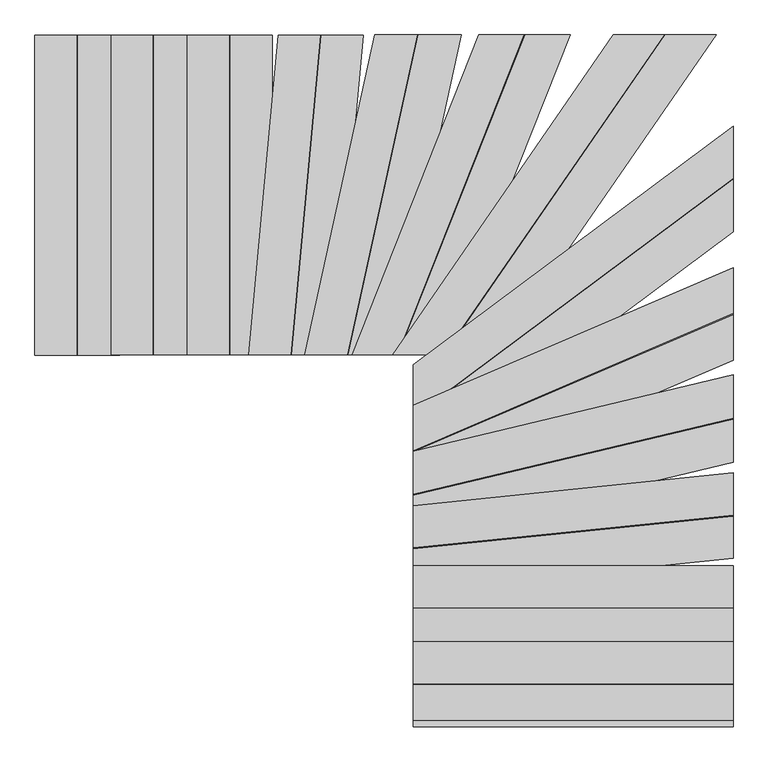
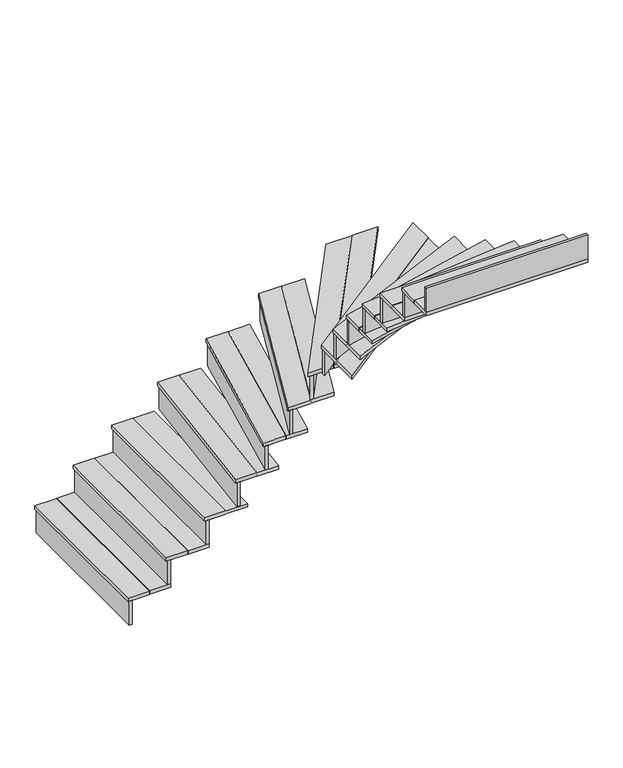
"""IFC4 building model written with IfcOpenShell, lengths in millimetres: stair flight geometry."""

from ifc_helpers import new_model, si_unit, origin, place, context, project, spatial, faceted_brep, source, transform, mapped, element, save


def stair_flight_5e1e636e(model_context):
    return source(origin(), model_context, "Body", "Brep", [
        faceted_brep([(-23979.400458, -9511.5570712, 168.402567), (-23979.400458, -9511.5570712, 0.0), (-23960.350458, -9511.5570712, 0.0), (-23960.350458, -9511.5570712, 168.402567), (-23979.400458, -8444.7570712, 168.402567), (-23960.350458, -8444.7570712, 168.402567), (-23960.350458, -8444.7570712, 0.0), (-23979.400458, -8444.7570712, 0.0)], [[[0, 1, 2, 3]], [[4, 5, 6, 7]], [[1, 0, 4, 7]], [[2, 1, 7, 6]], [[3, 2, 6, 5]], [[0, 3, 5, 4]]]),
        faceted_brep([(-23849.225458, -9511.5570712, 168.402567), (-23849.225458, -9511.5570712, 180.156839), (-23846.050458, -9511.5570712, 180.156839), (-23846.050458, -9511.5570712, 168.402567), (-23706.350458, -9511.5570712, 168.402567), (-23706.350458, -9511.5570712, 192.3142857), (-23846.050458, -9511.5570712, 192.3142857), (-23846.050458, -9511.5570712, 180.5600136), (-23849.225458, -9511.5570712, 180.5600136), (-23849.225458, -9511.5570712, 192.3142857), (-23988.925458, -9511.5570712, 192.3142857), (-23988.925458, -9511.5570712, 168.402567), (-23849.225458, -8444.7570712, 168.402567), (-23988.925458, -8444.7570712, 168.402567), (-23988.925458, -8444.7570712, 192.3142857), (-23849.225458, -8444.7570712, 192.3142857), (-23849.225458, -8444.7570712, 180.5600136), (-23846.050458, -8444.7570712, 180.5600136), (-23846.050458, -8444.7570712, 192.3142857), (-23706.350458, -8444.7570712, 192.3142857), (-23706.350458, -8444.7570712, 168.402567), (-23846.050458, -8444.7570712, 168.402567), (-23846.050458, -8444.7570712, 180.156839), (-23849.225458, -8444.7570712, 180.156839)], [[[0, 1, 2, 3, 4, 5, 6, 7, 8, 9, 10, 11]], [[12, 13, 14, 15, 16, 17, 18, 19, 20, 21, 22, 23]], [[1, 0, 12, 23]], [[2, 1, 23, 22]], [[3, 2, 22, 21]], [[4, 3, 21, 20]], [[5, 4, 20, 19]], [[6, 5, 19, 18]], [[7, 6, 18, 17]], [[8, 7, 17, 16]], [[9, 8, 16, 15]], [[10, 9, 15, 14]], [[11, 10, 14, 13]], [[0, 11, 13, 12]]]),
        faceted_brep([(-23725.400458, -9511.5570712, 360.7168527), (-23725.400458, -9511.5570712, 192.3142857), (-23706.350458, -9511.5570712, 192.3142857), (-23706.350458, -9511.5570712, 360.7168527), (-23725.400458, -8444.7570712, 360.7168527), (-23706.350458, -8444.7570712, 360.7168527), (-23706.350458, -8444.7570712, 192.3142857), (-23725.400458, -8444.7570712, 192.3142857)], [[[0, 1, 2, 3]], [[4, 5, 6, 7]], [[1, 0, 4, 7]], [[2, 1, 7, 6]], [[3, 2, 6, 5]], [[0, 3, 5, 4]]]),
        faceted_brep([(-23595.225458, -9511.5570712, 360.7168527), (-23595.225458, -9511.5570712, 372.4711248), (-23592.050458, -9511.5570712, 372.4711248), (-23592.050458, -9511.5570712, 360.7168527), (-23452.350458, -9511.5570712, 360.7168527), (-23452.350458, -9511.5570712, 384.6285714), (-23592.050458, -9511.5570712, 384.6285714), (-23592.050458, -9511.5570712, 372.8742994), (-23595.225458, -9511.5570712, 372.8742994), (-23595.225458, -9511.5570712, 384.6285714), (-23734.925458, -9511.5570712, 384.6285714), (-23734.925458, -9511.5570712, 360.7168527), (-23595.225458, -8444.7570712, 360.7168527), (-23734.925458, -8444.7570712, 360.7168527), (-23734.925458, -8444.7570712, 384.6285714), (-23595.225458, -8444.7570712, 384.6285714), (-23595.225458, -8444.7570712, 372.8742994), (-23592.050458, -8444.7570712, 372.8742994), (-23592.050458, -8444.7570712, 384.6285714), (-23452.350458, -8444.7570712, 384.6285714), (-23452.350458, -8444.7570712, 360.7168527), (-23592.050458, -8444.7570712, 360.7168527), (-23592.050458, -8444.7570712, 372.4711248), (-23595.225458, -8444.7570712, 372.4711248)], [[[0, 1, 2, 3, 4, 5, 6, 7, 8, 9, 10, 11]], [[12, 13, 14, 15, 16, 17, 18, 19, 20, 21, 22, 23]], [[1, 0, 12, 23]], [[2, 1, 23, 22]], [[3, 2, 22, 21]], [[4, 3, 21, 20]], [[5, 4, 20, 19]], [[6, 5, 19, 18]], [[7, 6, 18, 17]], [[8, 7, 17, 16]], [[9, 8, 16, 15]], [[10, 9, 15, 14]], [[11, 10, 14, 13]], [[0, 11, 13, 12]]]),
        faceted_brep([(-23471.400458, -9511.5570712, 553.0311384), (-23471.400458, -9511.5570712, 384.6285714), (-23452.350458, -9511.5570712, 384.6285714), (-23452.350458, -9511.5570712, 553.0311384), (-23471.400458, -8444.7570712, 553.0311384), (-23452.350458, -8444.7570712, 553.0311384), (-23452.350458, -8444.7570712, 384.6285714), (-23471.400458, -8444.7570712, 384.6285714)], [[[0, 1, 2, 3]], [[4, 5, 6, 7]], [[1, 0, 4, 7]], [[2, 1, 7, 6]], [[3, 2, 6, 5]], [[0, 3, 5, 4]]]),
        faceted_brep([(-23341.225458, -9511.5570712, 553.0311384), (-23341.225458, -9511.5570712, 564.7854105), (-23338.050458, -9511.5570712, 564.7854105), (-23338.050458, -9511.5570712, 553.0311384), (-23198.350458, -9511.5570712, 553.0311384), (-23198.350458, -9511.5570712, 576.9428571), (-23338.050458, -9511.5570712, 576.9428571), (-23338.050458, -9511.5570712, 565.1885851), (-23341.225458, -9511.5570712, 565.1885851), (-23341.225458, -9511.5570712, 576.9428571), (-23480.925458, -9511.5570712, 576.9428571), (-23480.925458, -9511.5570712, 553.0311384), (-23341.225458, -8444.7570712, 553.0311384), (-23480.925458, -8444.7570712, 553.0311384), (-23480.925458, -8444.7570712, 576.9428571), (-23341.225458, -8444.7570712, 576.9428571), (-23341.225458, -8444.7570712, 565.1885851), (-23338.050458, -8444.7570712, 565.1885851), (-23338.050458, -8444.7570712, 576.9428571), (-23198.350458, -8444.7570712, 576.9428571), (-23198.350458, -8444.7570712, 553.0311384), (-23338.050458, -8444.7570712, 553.0311384), (-23338.050458, -8444.7570712, 564.7854105), (-23341.225458, -8444.7570712, 564.7854105)], [[[0, 1, 2, 3, 4, 5, 6, 7, 8, 9, 10, 11]], [[12, 13, 14, 15, 16, 17, 18, 19, 20, 21, 22, 23]], [[1, 0, 12, 23]], [[2, 1, 23, 22]], [[3, 2, 22, 21]], [[4, 3, 21, 20]], [[5, 4, 20, 19]], [[6, 5, 19, 18]], [[7, 6, 18, 17]], [[8, 7, 17, 16]], [[9, 8, 16, 15]], [[10, 9, 15, 14]], [[11, 10, 14, 13]], [[0, 11, 13, 12]]]),
        faceted_brep([(-23267.1871269, -9511.5570712, 745.3454241), (-23267.1871269, -9511.5570712, 576.9428571), (-23248.0543246, -9511.5570712, 576.9428571), (-23248.0543246, -9511.5570712, 745.3454241), (-23167.6137891, -8444.7570712, 745.3454241), (-23148.4809868, -8444.7570712, 745.3454241), (-23148.4809868, -8444.7570712, 576.9428571), (-23167.6137891, -8444.7570712, 576.9428571)], [[[0, 1, 2, 3]], [[4, 5, 6, 7]], [[1, 0, 4, 7]], [[2, 1, 7, 6]], [[3, 2, 6, 5]], [[0, 3, 5, 4]]]),
        faceted_brep([(-23136.4463113, -9511.5570712, 745.3454241), (-23136.4463113, -9511.5570712, 757.0996962), (-23133.2575109, -9511.5570712, 757.0996962), (-23133.2575109, -9511.5570712, 745.3454241), (-22992.9502942, -9511.5570712, 745.3454241), (-22992.9502942, -9511.5570712, 769.2571429), (-23133.2575109, -9511.5570712, 769.2571429), (-23133.2575109, -9511.5570712, 757.5028708), (-23136.4463113, -9511.5570712, 757.5028708), (-23136.4463113, -9511.5570712, 769.2571429), (-23276.753528, -9511.5570712, 769.2571429), (-23276.753528, -9511.5570712, 745.3454241), (-23036.8729735, -8444.7570712, 745.3454241), (-23177.1801902, -8444.7570712, 745.3454241), (-23177.1801902, -8444.7570712, 769.2571429), (-23036.8729735, -8444.7570712, 769.2571429), (-23036.8729735, -8444.7570712, 757.5028708), (-23033.6841732, -8444.7570712, 757.5028708), (-23033.6841732, -8444.7570712, 769.2571429), (-22893.3769565, -8444.7570712, 769.2571429), (-22893.3769565, -8444.7570712, 745.3454241), (-23033.6841732, -8444.7570712, 745.3454241), (-23033.6841732, -8444.7570712, 757.0996962), (-23036.8729735, -8444.7570712, 757.0996962)], [[[0, 1, 2, 3, 4, 5, 6, 7, 8, 9, 10, 11]], [[12, 13, 14, 15, 16, 17, 18, 19, 20, 21, 22, 23]], [[1, 0, 12, 23]], [[2, 1, 23, 22]], [[3, 2, 22, 21]], [[4, 3, 21, 20]], [[5, 4, 20, 19]], [[6, 5, 19, 18]], [[7, 6, 18, 17]], [[8, 7, 17, 16]], [[9, 8, 16, 15]], [[10, 9, 15, 14]], [[11, 10, 14, 13]], [[0, 11, 13, 12]]]),
        faceted_brep([(-23080.0026813, -9511.5570712, 937.6597098), (-23080.0026813, -9511.5570712, 769.2571429), (-23060.502824, -9511.5570712, 769.2571429), (-23060.502824, -9511.5570712, 937.6597098), (-22846.7982346, -8444.7570712, 937.6597098), (-22827.2983773, -8444.7570712, 937.6597098), (-22827.2983773, -8444.7570712, 769.2571429), (-22846.7982346, -8444.7570712, 769.2571429)], [[[0, 1, 2, 3]], [[4, 5, 6, 7]], [[1, 0, 4, 7]], [[2, 1, 7, 6]], [[3, 2, 6, 5]], [[0, 3, 5, 4]]]),
        faceted_brep([(-22946.7536561, -9511.5570712, 937.6597098), (-22946.7536561, -9511.5570712, 949.4139819), (-22943.5036799, -9511.5570712, 949.4139819), (-22943.5036799, -9511.5570712, 937.6597098), (-22800.5047259, -9511.5570712, 937.6597098), (-22800.5047259, -9511.5570712, 961.5714286), (-22943.5036799, -9511.5570712, 961.5714286), (-22943.5036799, -9511.5570712, 949.8171565), (-22946.7536561, -9511.5570712, 949.8171565), (-22946.7536561, -9511.5570712, 961.5714286), (-23089.75261, -9511.5570712, 961.5714286), (-23089.75261, -9511.5570712, 937.6597098), (-22713.5492094, -8444.7570712, 937.6597098), (-22856.5481633, -8444.7570712, 937.6597098), (-22856.5481633, -8444.7570712, 961.5714286), (-22713.5492094, -8444.7570712, 961.5714286), (-22713.5492094, -8444.7570712, 949.8171565), (-22710.2992331, -8444.7570712, 949.8171565), (-22710.2992331, -8444.7570712, 961.5714286), (-22567.3002792, -8444.7570712, 961.5714286), (-22567.3002792, -8444.7570712, 937.6597098), (-22710.2992331, -8444.7570712, 937.6597098), (-22710.2992331, -8444.7570712, 949.4139819), (-22713.5492094, -8444.7570712, 949.4139819)], [[[0, 1, 2, 3, 4, 5, 6, 7, 8, 9, 10, 11]], [[12, 13, 14, 15, 16, 17, 18, 19, 20, 21, 22, 23]], [[1, 0, 12, 23]], [[2, 1, 23, 22]], [[3, 2, 22, 21]], [[4, 3, 21, 20]], [[5, 4, 20, 19]], [[6, 5, 19, 18]], [[7, 6, 18, 17]], [[8, 7, 17, 16]], [[9, 8, 16, 15]], [[10, 9, 15, 14]], [[11, 10, 14, 13]], [[0, 11, 13, 12]]]),
        faceted_brep([(-22920.2947085, -9511.5570712, 1129.9739955), (-22920.2947085, -9511.5570712, 961.5714286), (-22899.8081098, -9511.5570712, 961.5714286), (-22899.8081098, -9511.5570712, 1129.9739955), (-22498.2529462, -8444.7570712, 1129.9739955), (-22477.7663474, -8444.7570712, 1129.9739955), (-22477.7663474, -8444.7570712, 961.5714286), (-22498.2529462, -8444.7570712, 961.5714286)], [[[0, 1, 2, 3]], [[4, 5, 6, 7]], [[1, 0, 4, 7]], [[2, 1, 7, 6]], [[3, 2, 6, 5]], [[0, 3, 5, 4]]]),
        faceted_brep([(-22780.3029501, -9511.5570712, 1129.9739955), (-22780.3029501, -9511.5570712, 1141.7282676), (-22776.888517, -9511.5570712, 1141.7282676), (-22776.888517, -9511.5570712, 1129.9739955), (-22626.6534592, -9511.5570712, 1129.9739955), (-22626.6534592, -9511.5570712, 1153.8857143), (-22776.888517, -9511.5570712, 1153.8857143), (-22776.888517, -9511.5570712, 1142.1314422), (-22780.3029501, -9511.5570712, 1142.1314422), (-22780.3029501, -9511.5570712, 1153.8857143), (-22930.5380079, -9511.5570712, 1153.8857143), (-22930.5380079, -9511.5570712, 1129.9739955), (-22358.2611878, -8444.7570712, 1129.9739955), (-22508.4962456, -8444.7570712, 1129.9739955), (-22508.4962456, -8444.7570712, 1153.8857143), (-22358.2611878, -8444.7570712, 1153.8857143), (-22358.2611878, -8444.7570712, 1142.1314422), (-22354.8467546, -8444.7570712, 1142.1314422), (-22354.8467546, -8444.7570712, 1153.8857143), (-22204.6116968, -8444.7570712, 1153.8857143), (-22204.6116968, -8444.7570712, 1129.9739955), (-22354.8467546, -8444.7570712, 1129.9739955), (-22354.8467546, -8444.7570712, 1141.7282676), (-22358.2611878, -8444.7570712, 1141.7282676)], [[[0, 1, 2, 3, 4, 5, 6, 7, 8, 9, 10, 11]], [[12, 13, 14, 15, 16, 17, 18, 19, 20, 21, 22, 23]], [[1, 0, 12, 23]], [[2, 1, 23, 22]], [[3, 2, 22, 21]], [[4, 3, 21, 20]], [[5, 4, 20, 19]], [[6, 5, 19, 18]], [[7, 6, 18, 17]], [[8, 7, 17, 16]], [[9, 8, 16, 15]], [[10, 9, 15, 14]], [[11, 10, 14, 13]], [[0, 11, 13, 12]]]),
        faceted_brep([(-22784.9341182, -9511.5570712, 1322.2882812), (-22784.9341182, -9511.5570712, 1153.8857143), (-22761.7948561, -9511.5570712, 1153.8857143), (-22761.7948561, -9511.5570712, 1322.2882812), (-22049.3853628, -8444.7570712, 1322.2882812), (-22026.2461008, -8444.7570712, 1322.2882812), (-22026.2461008, -8444.7570712, 1153.8857143), (-22049.3853628, -8444.7570712, 1153.8857143)], [[[0, 1, 2, 3]], [[4, 5, 6, 7]], [[1, 0, 4, 7]], [[2, 1, 7, 6]], [[3, 2, 6, 5]], [[0, 3, 5, 4]]]),
        faceted_brep([(-22626.8158273, -9511.5570712, 1322.2882812), (-22626.8158273, -9511.5570712, 1334.0425533), (-22622.9592836, -9511.5570712, 1334.0425533), (-22622.9592836, -9511.5570712, 1322.2882812), (-22453.2713616, -9511.5570712, 1322.2882812), (-22453.2713616, -9511.5570712, 1346.2), (-22622.9592836, -9511.5570712, 1346.2), (-22622.9592836, -9511.5570712, 1334.4457279), (-22626.8158273, -9511.5570712, 1334.4457279), (-22626.8158273, -9511.5570712, 1346.2), (-22796.5037493, -9511.5570712, 1346.2), (-22796.5037493, -9511.5570712, 1322.2882812), (-21891.2670719, -8444.7570712, 1322.2882812), (-22060.9549939, -8444.7570712, 1322.2882812), (-22060.9549939, -8444.7570712, 1346.2), (-21891.2670719, -8444.7570712, 1346.2), (-21891.2670719, -8444.7570712, 1334.4457279), (-21887.4105282, -8444.7570712, 1334.4457279), (-21887.4105282, -8444.7570712, 1346.2), (-21717.7226062, -8444.7570712, 1346.2), (-21717.7226062, -8444.7570712, 1322.2882812), (-21887.4105282, -8444.7570712, 1322.2882812), (-21887.4105282, -8444.7570712, 1334.0425533), (-21891.2670719, -8444.7570712, 1334.0425533)], [[[0, 1, 2, 3, 4, 5, 6, 7, 8, 9, 10, 11]], [[12, 13, 14, 15, 16, 17, 18, 19, 20, 21, 22, 23]], [[1, 0, 12, 23]], [[2, 1, 23, 22]], [[3, 2, 22, 21]], [[4, 3, 21, 20]], [[5, 4, 20, 19]], [[6, 5, 19, 18]], [[7, 6, 18, 17]], [[8, 7, 17, 16]], [[9, 8, 16, 15]], [[10, 9, 15, 14]], [[11, 10, 14, 13]], [[0, 11, 13, 12]]]),
        faceted_brep([(-22727.8914763, -9555.4903958, 1514.602567), (-22727.8914763, -9555.4903958, 1346.2), (-22727.8914763, -9579.2511188, 1346.2), (-22727.8914763, -9579.2511188, 1514.602567), (-21661.0914763, -8760.2323116, 1514.602567), (-21661.0914763, -8783.9930346, 1514.602567), (-21661.0914763, -8783.9930346, 1346.2), (-21661.0914763, -8760.2323116, 1346.2)], [[[0, 1, 2, 3]], [[4, 5, 6, 7]], [[1, 0, 4, 7]], [[2, 1, 7, 6]], [[3, 2, 6, 5]], [[0, 3, 5, 4]]]),
        faceted_brep([(-22727.8914763, -9717.8553364, 1514.602567), (-22727.8914763, -9717.8553364, 1526.356839), (-22727.8914763, -9721.8154569, 1526.356839), (-22727.8914763, -9721.8154569, 1514.602567), (-22727.8914763, -9896.060759, 1514.602567), (-22727.8914763, -9896.060759, 1538.5142857), (-22727.8914763, -9721.8154569, 1538.5142857), (-22727.8914763, -9721.8154569, 1526.7600136), (-22727.8914763, -9717.8553364, 1526.7600136), (-22727.8914763, -9717.8553364, 1538.5142857), (-22727.8914763, -9543.6100343, 1538.5142857), (-22727.8914763, -9543.6100343, 1514.602567), (-21661.0914763, -8922.5972522, 1514.602567), (-21661.0914763, -8748.3519501, 1514.602567), (-21661.0914763, -8748.3519501, 1538.5142857), (-21661.0914763, -8922.5972522, 1538.5142857), (-21661.0914763, -8922.5972522, 1526.7600136), (-21661.0914763, -8926.5573727, 1526.7600136), (-21661.0914763, -8926.5573727, 1538.5142857), (-21661.0914763, -9100.8026748, 1538.5142857), (-21661.0914763, -9100.8026748, 1514.602567), (-21661.0914763, -8926.5573727, 1514.602567), (-21661.0914763, -8926.5573727, 1526.356839), (-21661.0914763, -8922.5972522, 1526.356839)], [[[0, 1, 2, 3, 4, 5, 6, 7, 8, 9, 10, 11]], [[12, 13, 14, 15, 16, 17, 18, 19, 20, 21, 22, 23]], [[1, 0, 12, 23]], [[2, 1, 23, 22]], [[3, 2, 22, 21]], [[4, 3, 21, 20]], [[5, 4, 20, 19]], [[6, 5, 19, 18]], [[7, 6, 18, 17]], [[8, 7, 17, 16]], [[9, 8, 16, 15]], [[10, 9, 15, 14]], [[11, 10, 14, 13]], [[0, 11, 13, 12]]]),
        faceted_brep([(-22727.8914763, -9689.5500482, 1706.9168527), (-22727.8914763, -9689.5500482, 1538.5142857), (-22727.8914763, -9710.2800893, 1538.5142857), (-22727.8914763, -9710.2800893, 1706.9168527), (-21661.0914763, -9231.7449787, 1706.9168527), (-21661.0914763, -9252.4750198, 1706.9168527), (-21661.0914763, -9252.4750198, 1538.5142857), (-21661.0914763, -9231.7449787, 1538.5142857)], [[[0, 1, 2, 3]], [[4, 5, 6, 7]], [[1, 0, 4, 7]], [[2, 1, 7, 6]], [[3, 2, 6, 5]], [[0, 3, 5, 4]]]),
        faceted_brep([(-22727.8914763, -9831.2053292, 1706.9168527), (-22727.8914763, -9831.2053292, 1718.6711248), (-22727.8914763, -9834.6603361, 1718.6711248), (-22727.8914763, -9834.6603361, 1706.9168527), (-22727.8914763, -9986.6806377, 1706.9168527), (-22727.8914763, -9986.6806377, 1730.8285714), (-22727.8914763, -9834.6603361, 1730.8285714), (-22727.8914763, -9834.6603361, 1719.0742994), (-22727.8914763, -9831.2053292, 1719.0742994), (-22727.8914763, -9831.2053292, 1730.8285714), (-22727.8914763, -9679.1850276, 1730.8285714), (-22727.8914763, -9679.1850276, 1706.9168527), (-21661.0914763, -9373.4002597, 1706.9168527), (-21661.0914763, -9221.3799581, 1706.9168527), (-21661.0914763, -9221.3799581, 1730.8285714), (-21661.0914763, -9373.4002597, 1730.8285714), (-21661.0914763, -9373.4002597, 1719.0742994), (-21661.0914763, -9376.8552666, 1719.0742994), (-21661.0914763, -9376.8552666, 1730.8285714), (-21661.0914763, -9528.8755682, 1730.8285714), (-21661.0914763, -9528.8755682, 1706.9168527), (-21661.0914763, -9376.8552666, 1706.9168527), (-21661.0914763, -9376.8552666, 1718.6711248), (-21661.0914763, -9373.4002597, 1718.6711248)], [[[0, 1, 2, 3, 4, 5, 6, 7, 8, 9, 10, 11]], [[12, 13, 14, 15, 16, 17, 18, 19, 20, 21, 22, 23]], [[1, 0, 12, 23]], [[2, 1, 23, 22]], [[3, 2, 22, 21]], [[4, 3, 21, 20]], [[5, 4, 20, 19]], [[6, 5, 19, 18]], [[7, 6, 18, 17]], [[8, 7, 17, 16]], [[9, 8, 16, 15]], [[10, 9, 15, 14]], [[11, 10, 14, 13]], [[0, 11, 13, 12]]]),
        faceted_brep([(-22727.8914763, -9843.0805325, 1899.2311384), (-22727.8914763, -9843.0805325, 1730.8285714), (-22727.8914763, -9862.6666989, 1730.8285714), (-22727.8914763, -9862.6666989, 1899.2311384), (-21661.0914763, -9588.2010846, 1899.2311384), (-21661.0914763, -9607.787251, 1899.2311384), (-21661.0914763, -9607.787251, 1730.8285714), (-21661.0914763, -9588.2010846, 1730.8285714)], [[[0, 1, 2, 3]], [[4, 5, 6, 7]], [[1, 0, 4, 7]], [[2, 1, 7, 6]], [[3, 2, 6, 5]], [[0, 3, 5, 4]]]),
        faceted_brep([(-22727.8914763, -9976.9193359, 1899.2311384), (-22727.8914763, -9976.9193359, 1910.9854105), (-22727.8914763, -9980.183697, 1910.9854105), (-22727.8914763, -9980.183697, 1899.2311384), (-22727.8914763, -10123.8155836, 1899.2311384), (-22727.8914763, -10123.8155836, 1923.1428571), (-22727.8914763, -9980.183697, 1923.1428571), (-22727.8914763, -9980.183697, 1911.3885851), (-22727.8914763, -9976.9193359, 1911.3885851), (-22727.8914763, -9976.9193359, 1923.1428571), (-22727.8914763, -9833.2874494, 1923.1428571), (-22727.8914763, -9833.2874494, 1899.2311384), (-21661.0914763, -9722.039888, 1899.2311384), (-21661.0914763, -9578.4080015, 1899.2311384), (-21661.0914763, -9578.4080015, 1923.1428571), (-21661.0914763, -9722.039888, 1923.1428571), (-21661.0914763, -9722.039888, 1911.3885851), (-21661.0914763, -9725.3042491, 1911.3885851), (-21661.0914763, -9725.3042491, 1923.1428571), (-21661.0914763, -9868.9361356, 1923.1428571), (-21661.0914763, -9868.9361356, 1899.2311384), (-21661.0914763, -9725.3042491, 1899.2311384), (-21661.0914763, -9725.3042491, 1910.9854105), (-21661.0914763, -9722.039888, 1910.9854105)], [[[0, 1, 2, 3, 4, 5, 6, 7, 8, 9, 10, 11]], [[12, 13, 14, 15, 16, 17, 18, 19, 20, 21, 22, 23]], [[1, 0, 12, 23]], [[2, 1, 23, 22]], [[3, 2, 22, 21]], [[4, 3, 21, 20]], [[5, 4, 20, 19]], [[6, 5, 19, 18]], [[7, 6, 18, 17]], [[8, 7, 17, 16]], [[9, 8, 16, 15]], [[10, 9, 15, 14]], [[11, 10, 14, 13]], [[0, 11, 13, 12]]]),
        faceted_brep([(-22727.8914763, -10024.3924621, 2091.5454241), (-22727.8914763, -10024.3924621, 1923.1428571), (-22727.8914763, -10043.5425575, 1923.1428571), (-22727.8914763, -10043.5425575, 2091.5454241), (-21661.0914763, -9914.889155, 2091.5454241), (-21661.0914763, -9934.0392504, 2091.5454241), (-21661.0914763, -9934.0392504, 1923.1428571), (-21661.0914763, -9914.889155, 1923.1428571)], [[[0, 1, 2, 3]], [[4, 5, 6, 7]], [[1, 0, 4, 7]], [[2, 1, 7, 6]], [[3, 2, 6, 5]], [[0, 3, 5, 4]]]),
        faceted_brep([(-22727.8914763, -10155.2514471, 2091.5454241), (-22727.8914763, -10155.2514471, 2103.2996962), (-22727.8914763, -10158.4431297, 2103.2996962), (-22727.8914763, -10158.4431297, 2091.5454241), (-22727.8914763, -10298.8771624, 2091.5454241), (-22727.8914763, -10298.8771624, 2115.4571429), (-22727.8914763, -10158.4431297, 2115.4571429), (-22727.8914763, -10158.4431297, 2103.7028708), (-22727.8914763, -10155.2514471, 2103.7028708), (-22727.8914763, -10155.2514471, 2115.4571429), (-22727.8914763, -10014.8174144, 2115.4571429), (-22727.8914763, -10014.8174144, 2091.5454241), (-21661.0914763, -10045.74814, 2091.5454241), (-21661.0914763, -9905.3141074, 2091.5454241), (-21661.0914763, -9905.3141074, 2115.4571429), (-21661.0914763, -10045.74814, 2115.4571429), (-21661.0914763, -10045.74814, 2103.7028708), (-21661.0914763, -10048.9398226, 2103.7028708), (-21661.0914763, -10048.9398226, 2115.4571429), (-21661.0914763, -10189.3738553, 2115.4571429), (-21661.0914763, -10189.3738553, 2091.5454241), (-21661.0914763, -10048.9398226, 2091.5454241), (-21661.0914763, -10048.9398226, 2103.2996962), (-21661.0914763, -10045.74814, 2103.2996962)], [[[0, 1, 2, 3, 4, 5, 6, 7, 8, 9, 10, 11]], [[12, 13, 14, 15, 16, 17, 18, 19, 20, 21, 22, 23]], [[1, 0, 12, 23]], [[2, 1, 23, 22]], [[3, 2, 22, 21]], [[4, 3, 21, 20]], [[5, 4, 20, 19]], [[6, 5, 19, 18]], [[7, 6, 18, 17]], [[8, 7, 17, 16]], [[9, 8, 16, 15]], [[10, 9, 15, 14]], [[11, 10, 14, 13]], [[0, 11, 13, 12]]]),
        faceted_brep([(-22727.8914763, -10223.6408086, 2283.8597098), (-22727.8914763, -10223.6408086, 2115.4571429), (-22727.8914763, -10242.6908086, 2115.4571429), (-22727.8914763, -10242.6908086, 2283.8597098), (-21661.0914763, -10223.6408086, 2283.8597098), (-21661.0914763, -10242.6908086, 2283.8597098), (-21661.0914763, -10242.6908086, 2115.4571429), (-21661.0914763, -10223.6408086, 2115.4571429)], [[[0, 1, 2, 3]], [[4, 5, 6, 7]], [[1, 0, 4, 7]], [[2, 1, 7, 6]], [[3, 2, 6, 5]], [[0, 3, 5, 4]]]),
        faceted_brep([(-22727.8914763, -10353.8158086, 2283.8597098), (-22727.8914763, -10353.8158086, 2295.6139819), (-22727.8914763, -10356.9908086, 2295.6139819), (-22727.8914763, -10356.9908086, 2283.8597098), (-22727.8914763, -10496.6908086, 2283.8597098), (-22727.8914763, -10496.6908086, 2307.7714286), (-22727.8914763, -10356.9908086, 2307.7714286), (-22727.8914763, -10356.9908086, 2296.0171565), (-22727.8914763, -10353.8158086, 2296.0171565), (-22727.8914763, -10353.8158086, 2307.7714286), (-22727.8914763, -10214.1158086, 2307.7714286), (-22727.8914763, -10214.1158086, 2283.8597098), (-21661.0914763, -10353.8158086, 2283.8597098), (-21661.0914763, -10214.1158086, 2283.8597098), (-21661.0914763, -10214.1158086, 2307.7714286), (-21661.0914763, -10353.8158086, 2307.7714286), (-21661.0914763, -10353.8158086, 2296.0171565), (-21661.0914763, -10356.9908086, 2296.0171565), (-21661.0914763, -10356.9908086, 2307.7714286), (-21661.0914763, -10496.6908086, 2307.7714286), (-21661.0914763, -10496.6908086, 2283.8597098), (-21661.0914763, -10356.9908086, 2283.8597098), (-21661.0914763, -10356.9908086, 2295.6139819), (-21661.0914763, -10353.8158086, 2295.6139819)], [[[0, 1, 2, 3, 4, 5, 6, 7, 8, 9, 10, 11]], [[12, 13, 14, 15, 16, 17, 18, 19, 20, 21, 22, 23]], [[1, 0, 12, 23]], [[2, 1, 23, 22]], [[3, 2, 22, 21]], [[4, 3, 21, 20]], [[5, 4, 20, 19]], [[6, 5, 19, 18]], [[7, 6, 18, 17]], [[8, 7, 17, 16]], [[9, 8, 16, 15]], [[10, 9, 15, 14]], [[11, 10, 14, 13]], [[0, 11, 13, 12]]]),
        faceted_brep([(-22727.8914763, -10477.6408086, 2476.1739955), (-22727.8914763, -10477.6408086, 2307.7714286), (-22727.8914763, -10496.6908086, 2307.7714286), (-22727.8914763, -10496.6908086, 2476.1739955), (-21661.0914763, -10477.6408086, 2476.1739955), (-21661.0914763, -10496.6908086, 2476.1739955), (-21661.0914763, -10496.6908086, 2307.7714286), (-21661.0914763, -10477.6408086, 2307.7714286)], [[[0, 1, 2, 3]], [[4, 5, 6, 7]], [[1, 0, 4, 7]], [[2, 1, 7, 6]], [[3, 2, 6, 5]], [[0, 3, 5, 4]]]),
        faceted_brep([(-22727.8914763, -10731.6408086, 2668.4882812), (-22727.8914763, -10731.6408086, 2500.0857143), (-22727.8914763, -10750.6908086, 2500.0857143), (-22727.8914763, -10750.6908086, 2668.4882812), (-21661.0914763, -10731.6408086, 2668.4882812), (-21661.0914763, -10750.6908086, 2668.4882812), (-21661.0914763, -10750.6908086, 2500.0857143), (-21661.0914763, -10731.6408086, 2500.0857143)], [[[0, 1, 2, 3]], [[4, 5, 6, 7]], [[1, 0, 4, 7]], [[2, 1, 7, 6]], [[3, 2, 6, 5]], [[0, 3, 5, 4]]]),
        faceted_brep([(-22727.8914763, -10607.8158086, 2476.1739955), (-22727.8914763, -10607.8158086, 2487.9282676), (-22727.8914763, -10610.9908086, 2487.9282676), (-22727.8914763, -10610.9908086, 2476.1739955), (-22727.8914763, -10750.6908086, 2476.1739955), (-22727.8914763, -10750.6908086, 2500.0857143), (-22727.8914763, -10610.9908086, 2500.0857143), (-22727.8914763, -10610.9908086, 2488.3314422), (-22727.8914763, -10607.8158086, 2488.3314422), (-22727.8914763, -10607.8158086, 2500.0857143), (-22727.8914763, -10468.1158086, 2500.0857143), (-22727.8914763, -10468.1158086, 2476.1739955), (-21661.0914763, -10607.8158086, 2476.1739955), (-21661.0914763, -10468.1158086, 2476.1739955), (-21661.0914763, -10468.1158086, 2500.0857143), (-21661.0914763, -10607.8158086, 2500.0857143), (-21661.0914763, -10607.8158086, 2488.3314422), (-21661.0914763, -10610.9908086, 2488.3314422), (-21661.0914763, -10610.9908086, 2500.0857143), (-21661.0914763, -10750.6908086, 2500.0857143), (-21661.0914763, -10750.6908086, 2476.1739955), (-21661.0914763, -10610.9908086, 2476.1739955), (-21661.0914763, -10610.9908086, 2487.9282676), (-21661.0914763, -10607.8158086, 2487.9282676)], [[[0, 1, 2, 3, 4, 5, 6, 7, 8, 9, 10, 11]], [[12, 13, 14, 15, 16, 17, 18, 19, 20, 21, 22, 23]], [[1, 0, 12, 23]], [[2, 1, 23, 22]], [[3, 2, 22, 21]], [[4, 3, 21, 20]], [[5, 4, 20, 19]], [[6, 5, 19, 18]], [[7, 6, 18, 17]], [[8, 7, 17, 16]], [[9, 8, 16, 15]], [[10, 9, 15, 14]], [[11, 10, 14, 13]], [[0, 11, 13, 12]]]),
    ])


if __name__ == "__main__":
    model = new_model("IFC4")
    model_context = context("Model", 3, world=origin())
    ifc_project = project(units=[si_unit("LENGTHUNIT", "METRE", prefix="MILLI")], contexts=[model_context])
    site = spatial("IfcSite", under=ifc_project)
    building = spatial("IfcBuilding", under=site)
    placement = place(None, origin())
    stair_flight_shape = stair_flight_5e1e636e(model_context)
    element("IfcStairFlight", 1, at=placement, inside=building, context=model_context, shape_type="MappedRepresentation", body=[
        mapped(stair_flight_shape, transform((0.0, 0.0, 0.0), x_axis=(1.0, 0.0, 0.0), y_axis=(0.0, 1.0, 0.0), z_axis=(0.0, 0.0, 1.0))),
    ])
    save(model, "model.ifc")

# Revit data of these elements
# Element 1 (IfcStairFlight)
#   Materials on its faces: "Composite Deck - Trex - Select - 1x6 Square Edge Board - Saddle - 20'"
# Materials
#   "Composite Deck - Trex - Select - 1x6 Square Edge Board - Saddle - 20'": class "Wood", colour RGB 120 75 45, transparency 0, Keynote = "06 11 00", Model = "Trex Select® Composite Deck 1\" Square Edge Board", Manufacturer = "Trex", URL = "http://www.trex.com/", Description = "1x6 Trex Select® Composite Deck Square Edge Board", Cost = 0
